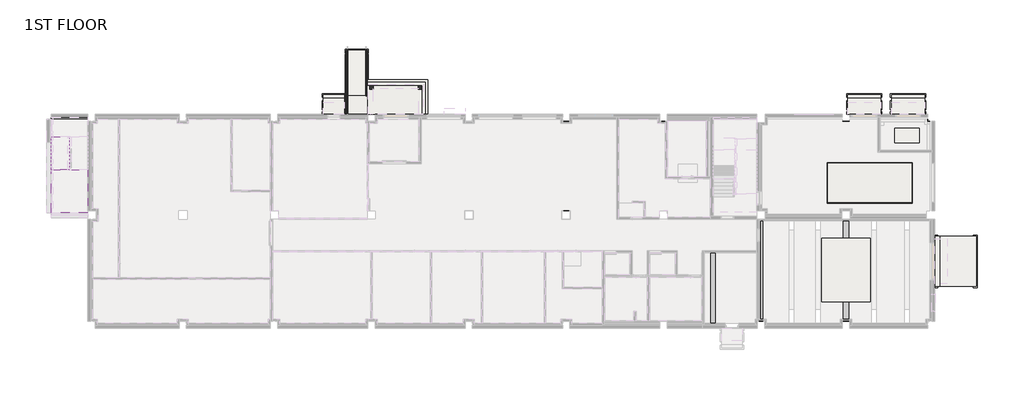
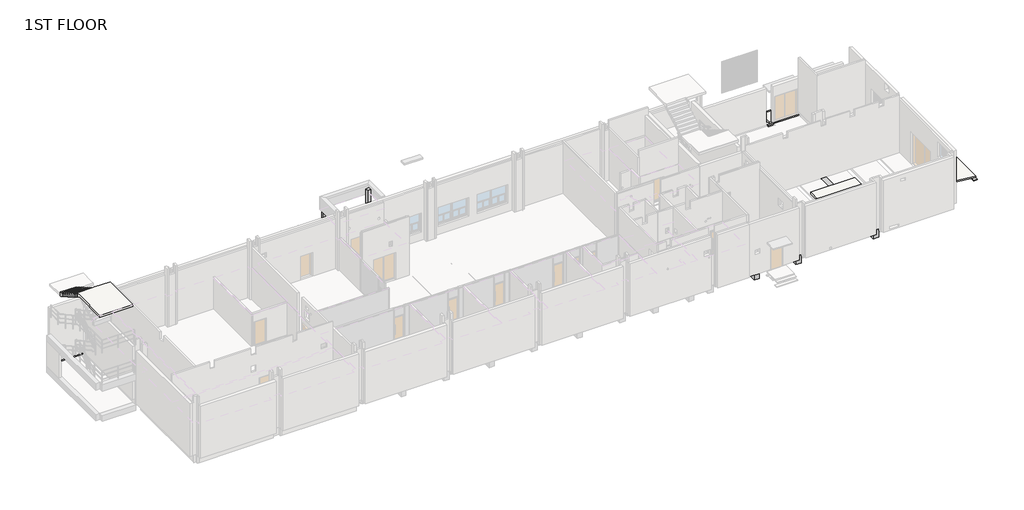
# One storey, part 10 of 15: 37 slabs, 9 beams, 2 columns, 1 stair flight.
"""IFC4 building model written with IfcOpenShell, lengths in millimetres."""

from ifc_helpers import new_model, si_unit, frame, origin, place, context, project, spatial, polyline, outline, extrude, faceted_brep, element, save

model = new_model("IFC4")

# Units and contexts
model_context = context("Model", 3, world=origin())
ifc_project = project(units=[si_unit("LENGTHUNIT", "METRE", prefix="MILLI")], contexts=[model_context])

# Site, building, storey
site = spatial("IfcSite", under=ifc_project)
building = spatial("IfcBuilding", under=site)
storey = spatial("IfcBuildingStorey", under=building, Name="1ST FLOOR", Elevation=4800.0)

# Beams
placement = place(None, origin())
element("IfcBeam", 1, ObjectType="RC Beam_Rectangular : H_SB_AR S16_TG-UG_500x800_1G2A", at=placement, inside=storey, context=model_context, shape_type="Brep", body=[
    faceted_brep([(47350.0, -8350.0, 4800.0), (50825.0, -8350.0, 4800.0), (50825.0, -7850.0, 4800.0), (47350.0, -7850.0, 4800.0), (47350.0, -8350.0, 4650.0), (47350.0, -8350.0, 4000.0), (50825.0, -8350.0, 4000.0), (50825.0, -8350.0, 4650.0), (47350.0, -7850.0, 4000.0), (50825.0, -7850.0, 4000.0), (50825.0, -7850.0, 4650.0), (47350.0, -7850.0, 4650.0)], [[[0, 1, 2, 3]], [[1, 0, 4, 5, 6, 7]], [[6, 5, 8, 9]], [[2, 10, 9, 8, 11, 3]], [[2, 1, 7, 6, 9, 10]], [[8, 5, 4, 0, 3, 11]]]),
])
element("IfcBeam", 2, ObjectType="RC Beam_Rectangular : H_SB_AR S16_TG-UG_500x800_1G1", at=placement, inside=storey, context=model_context, shape_type="Brep", body=[
    faceted_brep([(39250.0, -300.0, 4800.0), (38750.0, -300.0, 4800.0), (38750.0, -7650.0, 4800.0), (39250.0, -7650.0, 4800.0), (39250.0, -7650.0, 4650.0), (39250.0, -7650.0, 4000.0), (39250.0, -300.0, 4000.0), (39250.0, -300.0, 4650.0), (38750.0, -300.0, 4000.0), (38750.0, -7650.0, 4000.0), (38750.0, -300.0, 4650.0), (38750.0, -7650.0, 4650.0)], [[[0, 1, 2, 3]], [[0, 3, 4, 5, 6, 7]], [[8, 6, 5, 9]], [[2, 1, 10, 8, 9, 11]], [[1, 0, 7, 6, 8, 10]], [[3, 2, 11, 9, 5, 4]]]),
])
element("IfcBeam", 3, ObjectType="RC Beam_Rectangular : H_SB_AR S16_TG-UG_500x800_1G1", at=placement, inside=storey, context=model_context, shape_type="Brep", body=[
    faceted_brep([(47300.0, -300.0, 4800.0), (47150.0, -300.0, 4800.0), (46800.0, -300.0, 4800.0), (46800.0, -7650.0, 4800.0), (47300.0, -7650.0, 4800.0), (47300.0, -4975.0, 4800.0), (47300.0, -4825.0, 4800.0), (47300.0, -300.0, 4000.0), (47300.0, -7650.0, 4650.0), (47300.0, -7650.0, 4000.0), (46800.0, -300.0, 4000.0), (46800.0, -7650.0, 4000.0), (46800.0, -300.0, 4650.0), (46800.0, -7650.0, 4650.0)], [[[0, 1, 2, 3, 4, 5, 6]], [[7, 0, 6, 5, 4, 8, 9]], [[10, 7, 9, 11]], [[3, 2, 12, 10, 11, 13]], [[2, 1, 0, 7, 10, 12]], [[4, 3, 13, 11, 9, 8]]]),
])
element("IfcBeam", 4, ObjectType="RC Beam_Rectangular : H_SB_AR S16_TG-UG_450x800_1B1", at=placement, inside=storey, context=model_context, shape_type="Brep", body=[
    faceted_brep([(42125.0, -100.0, 4800.0), (41675.0, -100.0, 4800.0), (41675.0, -7850.0, 4800.0), (42125.0, -7850.0, 4800.0), (42125.0, -7850.0, 4650.0), (42125.0, -7850.0, 4000.0), (42125.0, -100.0, 4000.0), (42125.0, -100.0, 4650.0), (41675.0, -100.0, 4000.0), (41675.0, -7850.0, 4000.0), (41675.0, -100.0, 4650.0), (41675.0, -7850.0, 4650.0)], [[[0, 1, 2, 3]], [[0, 3, 4, 5, 6, 7]], [[8, 6, 5, 9]], [[2, 1, 10, 8, 9, 11]], [[1, 0, 7, 6, 8, 10]], [[3, 2, 11, 9, 5, 4]]]),
])
element("IfcBeam", 5, ObjectType="RC Beam_Rectangular : H_SB_AR S16_TG-UG_450x800_1B1", at=placement, inside=storey, context=model_context, shape_type="Brep", body=[
    faceted_brep([(45325.0, -100.0, 4800.0), (44875.0, -100.0, 4800.0), (44875.0, -7850.0, 4800.0), (45325.0, -7850.0, 4800.0), (45325.0, -7850.0, 4650.0), (45325.0, -7850.0, 4000.0), (45325.0, -100.0, 4000.0), (45325.0, -100.0, 4650.0), (44875.0, -100.0, 4000.0), (44875.0, -7850.0, 4000.0), (44875.0, -100.0, 4650.0), (44875.0, -7850.0, 4650.0)], [[[0, 1, 2, 3]], [[0, 3, 4, 5, 6, 7]], [[8, 6, 5, 9]], [[2, 1, 10, 8, 9, 11]], [[1, 0, 7, 6, 8, 10]], [[3, 2, 11, 9, 5, 4]]]),
])
element("IfcBeam", 6, ObjectType="RC Beam_Rectangular : H_SB_AR S16_TG-UG_450x800_1B1A", at=placement, inside=storey, context=model_context, shape_type="Brep", body=[
    faceted_brep([(50825.0, -8350.0, 4800.0), (51275.0, -8350.0, 4800.0), (51275.0, -8350.0, 4650.0), (51275.0, -8350.0, 4000.0), (50825.0, -8350.0, 4000.0), (50825.0, -8350.0, 4650.0), (50825.0, -16900.0, 4800.0), (51275.0, -16900.0, 4800.0), (51275.0, -16900.0, 4650.0), (51275.0, -16900.0, 4000.0), (50825.0, -16900.0, 4000.0), (50825.0, -15750.0000001, 4000.0), (50825.0, -16900.0, 4650.0)], [[[0, 1, 2, 3, 4, 5]], [[1, 0, 6, 7]], [[1, 7, 8, 9, 3, 2]], [[4, 3, 9, 10, 11]], [[6, 0, 5, 4, 11, 10, 12]], [[7, 6, 12, 10, 9, 8]]]),
])
element("IfcBeam", 7, ObjectType="RC Beam_Rectangular : H_SB_AR S16_TG-UG_500x800_1G1", at=placement, inside=storey, context=model_context, shape_type="Brep", body=[
    faceted_brep([(55200.0, -8350.0, 4800.0), (54700.0, -8350.0, 4800.0), (54700.0, -16700.0, 4800.0), (55200.0, -16700.0, 4800.0), (55200.0, -16700.0, 4650.0), (55200.0, -16700.0, 4000.0), (55200.0, -8350.0, 4000.0), (55200.0, -8350.0, 4650.0), (54700.0, -8350.0, 4000.0), (54700.0, -16700.0, 4000.0), (54700.0, -8350.0, 4650.0), (54700.0, -16700.0, 4650.0)], [[[0, 1, 2, 3]], [[0, 3, 4, 5, 6, 7]], [[8, 6, 5, 9]], [[2, 1, 10, 8, 9, 11]], [[1, 0, 7, 6, 8, 10]], [[3, 2, 11, 9, 5, 4]]]),
])
element("IfcBeam", 8, ObjectType="RC Beam_Rectangular : H_SB_AR S16_TG-UG_500x800_1G1", at=placement, inside=storey, context=model_context, shape_type="Brep", body=[
    faceted_brep([(62250.0, -8350.0, 4800.0), (61750.0, -8350.0, 4800.0), (61750.0, -16700.0, 4800.0), (62250.0, -16700.0, 4800.0), (62250.0, -16700.0, 4650.0), (62250.0, -16700.0, 4000.0), (62250.0, -8350.0, 4000.0), (62250.0, -8350.0, 4650.0), (61750.0, -8350.0, 4000.0), (61750.0, -16700.0, 4000.0), (61750.0, -8350.0, 4650.0), (61750.0, -16700.0, 4650.0)], [[[0, 1, 2, 3]], [[0, 3, 4, 5, 6, 7]], [[8, 6, 5, 9]], [[2, 1, 10, 8, 9, 11]], [[1, 0, 7, 6, 8, 10]], [[3, 2, 11, 9, 5, 4]]]),
])
element("IfcBeam", 9, ObjectType="RC Beam_Rectangular : H_SB_AR S16_RC Beam-AG_400x530_SG1A", at=placement, inside=storey, context=model_context, shape_type="Brep", body=[
    faceted_brep([(-300.0, -100.0, 4630.0), (-300.0, 50.0, 4630.0), (-300.0, 300.0, 4630.0), (-3300.0, 300.0, 4630.0), (-3300.0, 50.0, 4630.0), (-3300.0, -100.0, 4630.0), (-300.0, -100.0, 4100.0), (-300.0, -100.0, 4430.0), (-3300.0, -100.0, 4430.0), (-3300.0, -100.0, 4100.0), (-300.0, 300.0, 4100.0), (-3300.0, 300.0, 4100.0)], [[[0, 1, 2, 3, 4, 5]], [[6, 7, 0, 5, 8, 9]], [[10, 6, 9, 11]], [[2, 10, 11, 3]], [[2, 1, 0, 7, 6, 10]], [[3, 11, 9, 8, 5, 4]]]),
])

# Columns
element("IfcColumn", 10, ObjectType="RC_Column_Rectangular : H_SC_AR S15_RC Col-AG_300x300_C4", at=placement, inside=storey, context=model_context, shape_type="Brep", body=[
    faceted_brep([(23150.0, 2650.0, 4585.0), (23150.0, 2620.0, 4585.0), (23150.0, 2350.0, 4585.0), (22850.0, 2350.0, 4585.0), (22850.0, 2620.0, 4585.0), (22850.0, 2650.0, 4585.0), (23150.0, 2650.0, 9300.0), (23150.0, 2350.0, 9300.0), (23150.0, 2350.0, 4750.0), (22850.0, 2350.0, 9300.0), (22850.0, 2350.0, 4750.0), (22850.0, 2650.0, 9300.0), (23000.0, 2650.0, 9300.0)], [[[0, 1, 2, 3, 4, 5]], [[6, 7, 8, 2, 1, 0]], [[7, 9, 10, 3, 2, 8]], [[9, 11, 5, 4, 3, 10]], [[11, 12, 6, 0, 5]], [[6, 12, 11, 9, 7]]]),
])
element("IfcColumn", 11, ObjectType="RC_Column_Rectangular : H_SC_AR S15_RC Col-AG_300x300_C4", at=placement, inside=storey, context=model_context, shape_type="Brep", body=[
    faceted_brep([(27150.0, 2650.0, 4585.0), (27150.0, 2350.0, 4585.0), (27120.0, 2350.0, 4585.0), (26850.0, 2350.0, 4585.0), (26850.0, 2620.0, 4585.0), (26850.0, 2650.0, 4585.0), (27150.0, 2650.0, 9300.0), (27150.0, 2500.0, 9300.0), (27150.0, 2350.0, 9300.0), (26850.0, 2350.0, 9300.0), (26850.0, 2350.0, 4750.0), (26850.0, 2650.0, 9300.0)], [[[0, 1, 2, 3, 4, 5]], [[6, 7, 8, 1, 0]], [[8, 9, 10, 3, 2, 1]], [[9, 11, 5, 4, 3, 10]], [[11, 6, 0, 5]], [[6, 11, 9, 8, 7]]]),
])

# Slabs
element("IfcSlab", 12, ObjectType="H_SF_AR S18_MAT_T650_MF2", at=placement, inside=storey, context=model_context, shape_type="Brep", body=[
    faceted_brep([(27625.0, 3125.0000075, 4100.0), (27625.0, 300.0, 4100.0), (22650.0, 300.0, 4100.0), (22650.0, 3125.0000075, 4100.0), (22650.0, 300.0, 4750.0), (27120.0, 300.0, 4750.0), (27120.0, 2350.0, 4750.0), (26850.0, 2350.0, 4750.0), (26850.0, 2620.0, 4750.0), (23150.0, 2620.0, 4750.0), (23150.0, 2350.0, 4750.0), (22850.0, 2350.0, 4750.0), (22850.0, 2620.0, 4750.0), (22650.0, 2620.0, 4750.0), (27625.0, 3125.0000075, 4500.0), (27625.0, 300.0, 4500.0), (27420.0, 300.0, 4500.0), (27420.0, 300.0, 4585.0), (27120.0, 300.0, 4585.0), (22650.0, 300.0, 4500.0), (22650.0, 300.0, 4450.0), (22650.0, 300.0, 4400.0), (22650.0, 2620.0, 4585.0), (22650.0, 2920.0, 4585.0), (22650.0, 2920.0, 4500.0), (22650.0, 3125.0000075, 4500.0), (22650.0, 3125.0000075, 4361.6666662), (22650.0, 3125.0000075, 4311.5556782), (27420.0, 2920.0, 4585.0), (22850.0, 2620.0, 4585.0), (22850.0, 2350.0, 4585.0), (23150.0, 2350.0, 4585.0), (23150.0, 2620.0, 4585.0), (26850.0, 2620.0, 4585.0), (26850.0, 2350.0, 4585.0), (27120.0, 2350.0, 4585.0), (27420.0, 2920.0, 4500.0)], [[[0, 1, 2, 3]], [[4, 5, 6, 7, 8, 9, 10, 11, 12, 13]], [[1, 0, 14, 15]], [[2, 1, 15, 16, 17, 18, 5, 4, 19, 20, 21]], [[3, 2, 21, 20, 19, 4, 13, 22, 23, 24, 25, 26, 27]], [[0, 3, 27, 26, 25, 14]], [[17, 28, 23, 22, 29, 30, 31, 32, 33, 34, 35, 18]], [[28, 17, 16, 36]], [[36, 16, 15, 14, 25, 24]], [[5, 18, 35, 6]], [[23, 28, 36, 24]], [[8, 33, 32, 9]], [[22, 13, 12, 29]], [[35, 34, 7, 6]], [[34, 33, 8, 7]], [[32, 31, 10, 9]], [[31, 30, 11, 10]], [[30, 29, 12, 11]]]),
])
element("IfcSlab", 13, ObjectType="H_SF_AR B01_EQ Fdn_T800_EF1", at=placement, inside=storey, context=model_context, shape_type="Brep", body=[
    faceted_brep([(60500.0, -3750.0, 4200.0), (67400.0, -3750.0, 4200.0), (67400.0, -6950.0, 4200.0), (60500.0, -6950.0, 4200.0), (60500.0, -3750.0, 5000.0), (60500.0, -6950.0, 5000.0), (67400.0, -6950.0, 5000.0), (67400.0, -3750.0, 5000.0), (60500.0, -3750.0, 4600.0), (60500.0, -3750.0, 4650.0), (67400.0, -3750.0, 4650.0), (67400.0, -3750.0, 4600.0), (67400.0, -6950.0, 4650.0), (67400.0, -6950.0, 4600.0), (60500.0, -6950.0, 4650.0), (60500.0, -6950.0, 4600.0)], [[[0, 1, 2, 3]], [[4, 5, 6, 7]], [[1, 0, 8, 9, 4, 7, 10, 11]], [[2, 1, 11, 10, 7, 6, 12, 13]], [[3, 2, 13, 12, 6, 5, 14, 15]], [[0, 3, 15, 14, 5, 4, 9, 8]]]),
])
element("IfcSlab", 14, ObjectType="H_SF_AR B01_EQ Fdn_T200_EF2", at=placement, inside=storey, context=model_context, shape_type="SweptSolid", body=[
    extrude(outline(polyline([(64000.0000005, -9900.0), (64000.0000005, -15100.0), (59999.9999995, -15100.0), (59999.9999995, -9900.0), (64000.0000005, -9900.0)])), frame((0.0, 0.0, 4800.0), z_axis=(0.0, 0.0, 1.0), x_axis=(1.0, 0.0, 0.0)), (0.0, 0.0, 1.0), 200.0),
])
element("IfcSlab", 15, ObjectType="H_SF_AR B01_EQ Fdn_T200_EF3", at=placement, inside=storey, context=model_context, shape_type="SweptSolid", body=[
    extrude(outline(polyline([(66000.0, -850.0), (68000.0, -850.0), (68000.0, -2050.0), (66000.0, -2050.0), (66000.0, -850.0)])), frame((0.0, 0.0, 4800.0), z_axis=(0.0, 0.0, 1.0), x_axis=(1.0, 0.0, 0.0)), (0.0, 0.0, 1.0), 200.0),
])
element("IfcSlab", 16, ObjectType="H_FL_AR_S17_RC Slab_T200_SS1", at=placement, inside=storey, context=model_context, shape_type="Brep", body=[
    faceted_brep([(-1850.0, -4250.0, 14050.0), (-3300.0, -4250.0, 14050.0), (-3300.0, -4604.0698283, 14050.0), (-3300.0, -7800.0, 14050.0), (-300.0, -7800.0, 14050.0), (-300.0, -4250.0, 14050.0), (-1750.0, -4250.0, 14050.0), (-1850.0, -4250.0, 13850.0), (-1850.0, -4250.0, 13643.4592668), (-3300.0, -4250.0, 13643.4592668), (-3300.0, -4604.0698283, 13850.0), (-3300.0, -7800.0, 13850.0), (-300.0, -7800.0, 13850.0), (-300.0, -4250.0, 13850.0), (-1750.0, -4250.0, 13850.0), (-1850.0, -4604.0698283, 13850.0)], [[[0, 1, 2, 3, 4, 5, 6]], [[1, 0, 7, 8, 9]], [[1, 9, 10, 11, 3, 2]], [[4, 3, 11, 12]], [[5, 4, 12, 13]], [[0, 6, 14, 7]], [[10, 15, 7, 14, 13, 12, 11]], [[15, 10, 9, 8]], [[7, 15, 8]], [[6, 5, 13, 14]]]),
])
element("IfcSlab", 17, ObjectType="H_SF_AR_B08_Ramp_T150", at=placement, inside=storey, context=model_context, shape_type="SweptSolid", body=[
    extrude(outline(polyline([(69700.0, -9750.0), (69700.0, -13850.0), (69312.0, -13850.0), (69312.0, -9750.0), (69700.0, -9750.0)])), frame((0.0, 0.0, 4650.0), z_axis=(0.0, 0.0, 1.0), x_axis=(1.0, 0.0, 0.0)), (0.0, 0.0, 1.0), 150.0),
])
element("IfcSlab", 18, ObjectType="H_SF_AR_B08_Ramp_T150", at=placement, inside=storey, context=model_context, shape_type="Brep", body=[
    faceted_brep([(72700.0, -9750.0, 4349.2518657), (72700.0, -10050.0, 4349.2518657), (72700.0, -13550.0, 4349.2518657), (72700.0, -13850.0, 4349.2518657), (72256.3868159, -13850.0, 4393.6131841), (72256.3868159, -13550.0, 4393.6131841), (72256.3868159, -10050.0, 4393.6131841), (72256.3868159, -9750.0, 4393.6131841), (69700.0, -10050.0, 4649.2518657), (69700.0, -9750.0, 4649.2518657), (72250.0, -9750.0, 4394.2518657), (72250.0, -10050.0, 4394.2518657), (72250.0, -13550.0, 4394.2518657), (72250.0, -13850.0, 4394.2518657), (69700.0, -13850.0, 4649.2518657), (69700.0, -13550.0, 4649.2518657), (72700.0, -13850.0, 4500.0), (72700.0, -9750.0, 4500.0), (69700.0, -9750.0, 4800.0), (69700.0, -13850.0, 4800.0), (69700.0, -13850.0, 4650.0), (72250.0, -13850.0, 4400.0), (69700.0, -9750.0, 4650.0), (72250.0, -9750.0, 4400.0)], [[[0, 1, 2, 3, 4, 5, 6, 7]], [[8, 9, 10, 11, 12, 13, 14, 15]], [[16, 17, 18, 19]], [[17, 16, 3, 2, 1, 0]], [[16, 19, 20, 14, 13, 21, 4, 3]], [[19, 18, 22, 9, 8, 15, 14, 20]], [[18, 17, 0, 7, 23, 10, 9, 22]], [[21, 23, 7, 6, 5, 4]], [[23, 21, 13, 12, 11, 10]]]),
])
element("IfcSlab", 19, ObjectType="H_SF_AR_S18_Lean_T50", at=placement, inside=storey, context=model_context, shape_type="SweptSolid", body=[
    extrude(outline(polyline([(69550.0, -9650.0), (69550.0, -13950.0), (69300.0, -13950.0), (69300.0, -9650.0), (69550.0, -9650.0)])), frame((0.0, 0.0, 4450.0), z_axis=(0.0, 0.0, 1.0), x_axis=(1.0, 0.0, 0.0)), (0.0, 0.0, 1.0), 50.0),
])
element("IfcSlab", 20, ObjectType="H_SF_AR_S18_Lean_T50", at=placement, inside=storey, context=model_context, shape_type="SweptSolid", body=[
    extrude(outline(polyline([(72450.0, -9650.0), (72800.0, -9650.0), (72800.0, -13950.0), (72450.0, -13950.0), (72450.0, -9650.0)])), frame((0.0, 0.0, 4150.0), z_axis=(0.0, 0.0, 1.0), x_axis=(1.0, 0.0, 0.0)), (0.0, 0.0, 1.0), 50.0),
])
element("IfcSlab", 21, ObjectType="H_SF_AR_S18_Lean_T50", at=placement, inside=storey, context=model_context, shape_type="Brep", body=[
    faceted_brep([(69700.0, -13550.0, 4599.0024876), (69700.0, -10050.0, 4599.0024876), (69717.9210597, -10050.0, 4597.2103816), (72233.6520381, -10050.0, 4345.6372838), (72233.6520381, -13550.0, 4345.6372838), (69717.9210597, -13550.0, 4597.2103816), (69700.0, -10050.0, 4649.2518657), (69700.0, -13550.0, 4649.2518657), (72250.0, -13550.0, 4394.2518657), (72250.0, -10050.0, 4394.2518657), (69700.0, -13550.0, 4600.0), (72229.2893219, -13550.0, 4350.0), (72250.0, -13550.0, 4350.0), (69700.0, -10050.0, 4600.0), (72250.0, -10050.0, 4350.0), (72229.2893219, -10050.0, 4350.0)], [[[0, 1, 2, 3, 4, 5]], [[6, 7, 8, 9]], [[7, 10, 0, 5, 4, 11, 12, 8]], [[1, 0, 10, 7, 6, 13]], [[1, 13, 6, 9, 14, 15, 3, 2]], [[15, 11, 4, 3]], [[11, 15, 14, 12]], [[12, 14, 9, 8]]]),
])
element("IfcSlab", 22, ObjectType="H_SF_AR_B08_Ramp_T150", at=placement, inside=storey, context=model_context, shape_type="Brep", body=[
    faceted_brep([(22638.0, 1800.0, 4600.0), (22638.0, 312.0, 4600.0), (22338.0, 312.0, 4600.0), (21238.0, 312.0, 4600.0), (20938.0, 312.0, 4600.0), (20938.0, 1800.0, 4600.0), (22638.0, 1800.0, 4750.0), (20938.0, 1800.0, 4750.0), (20938.0, 312.0, 4750.0), (22638.0, 312.0, 4750.0)], [[[0, 1, 2, 3, 4, 5]], [[6, 7, 8, 9]], [[1, 0, 6, 9]], [[4, 3, 2, 1, 9, 8]], [[5, 4, 8, 7]], [[0, 5, 7, 6]]]),
])
element("IfcSlab", 23, ObjectType="H_SF_AR_B08_Stoop_T150", at=placement, inside=storey, context=model_context, shape_type="Brep", body=[
    faceted_brep([(68450.0, 1600.0, 4600.0), (68450.0, 1400.0, 4600.0), (68450.0, 662.0000074, 4600.0), (68450.0, 312.0000074, 4600.0), (65750.0, 312.0000074, 4600.0), (65750.0, 662.0000074, 4600.0), (65750.0, 1400.0, 4600.0), (65750.0, 1600.0, 4600.0), (68450.0, 1600.0, 4750.0), (65750.0, 1600.0, 4750.0), (65750.0, 312.0000074, 4750.0), (68450.0, 312.0000074, 4750.0), (68450.0, 1600.0, 4625.0), (65750.0, 1600.0, 4625.0)], [[[0, 1, 2, 3, 4, 5, 6, 7]], [[8, 9, 10, 11]], [[3, 2, 1, 0, 12, 8, 11]], [[4, 3, 11, 10]], [[7, 6, 5, 4, 10, 9, 13]], [[0, 7, 13, 9, 8, 12]]]),
])
element("IfcSlab", 24, ObjectType="H_SF_AR_B08_Stoop_T125", at=placement, inside=storey, context=model_context, shape_type="SweptSolid", body=[
    extrude(outline(polyline([(68450.0, 1900.0), (68450.0, 1600.0), (65750.0, 1600.0), (65750.0, 1900.0), (68450.0, 1900.0)])), frame((0.0, 0.0, 4600.0), z_axis=(0.0, 0.0, 1.0), x_axis=(1.0, 0.0, 0.0)), (0.0, 0.0, 1.0), 25.0),
])
element("IfcSlab", 25, ObjectType="H_SF_AR_S18_Lean_T50", at=placement, inside=storey, context=model_context, shape_type="SweptSolid", body=[
    extrude(outline(polyline([(68550.0, 2000.0), (68550.0, 1700.0), (65650.0, 1700.0), (65650.0, 2000.0), (68550.0, 2000.0)])), frame((0.0, 0.0, 4250.0), z_axis=(0.0, 0.0, 1.0), x_axis=(1.0, 0.0, 0.0)), (0.0, 0.0, 1.0), 50.0),
])
element("IfcSlab", 26, ObjectType="H_SF_AR_S18_Lean_T50", at=placement, inside=storey, context=model_context, shape_type="SweptSolid", body=[
    extrude(outline(polyline([(68550.0, 300.0), (65650.0, 300.0), (65650.0, 512.0000074), (68550.0, 512.0000074), (68550.0, 300.0)])), frame((0.0, 0.0, 4400.0), z_axis=(0.0, 0.0, 1.0), x_axis=(1.0, 0.0, 0.0)), (0.0, 0.0, 1.0), 50.0),
])
element("IfcSlab", 27, ObjectType="H_SF_AR_S18_Lean_T50", at=placement, inside=storey, context=model_context, shape_type="Brep", body=[
    faceted_brep([(68550.0, 1400.0, 4550.0), (68550.0, 1379.2893219, 4550.0), (68550.0, 682.7106855, 4550.0), (68550.0, 662.0000074, 4550.0), (65650.0, 662.0000074, 4550.0), (65650.0, 682.7106855, 4550.0), (65650.0, 1379.2893219, 4550.0), (65650.0, 1400.0, 4550.0), (68550.0, 1400.0, 4600.0), (65650.0, 1400.0, 4600.0), (65650.0, 662.0000074, 4600.0), (68550.0, 662.0000074, 4600.0)], [[[0, 1, 2, 3, 4, 5, 6, 7]], [[8, 9, 10, 11]], [[3, 2, 1, 0, 8, 11]], [[4, 3, 11, 10]], [[7, 6, 5, 4, 10, 9]], [[0, 7, 9, 8]]]),
])
element("IfcSlab", 28, ObjectType="H_SF_AR_B08_Stoop_T150", at=placement, inside=storey, context=model_context, shape_type="Brep", body=[
    faceted_brep([(64850.0, 1600.0, 4600.0), (64850.0, 1400.0, 4600.0), (64850.0, 662.0000074, 4600.0), (64850.0, 312.0000074, 4600.0), (62150.0, 312.0000074, 4600.0), (62150.0, 662.0000074, 4600.0), (62150.0, 1400.0, 4600.0), (62150.0, 1600.0, 4600.0), (64850.0, 1600.0, 4750.0), (62150.0, 1600.0, 4750.0), (62150.0, 312.0000074, 4750.0), (64850.0, 312.0000074, 4750.0), (64850.0, 1600.0, 4625.0), (62150.0, 1600.0, 4625.0)], [[[0, 1, 2, 3, 4, 5, 6, 7]], [[8, 9, 10, 11]], [[3, 2, 1, 0, 12, 8, 11]], [[4, 3, 11, 10]], [[7, 6, 5, 4, 10, 9, 13]], [[0, 7, 13, 9, 8, 12]]]),
])
element("IfcSlab", 29, ObjectType="H_SF_AR_B08_Stoop_T125", at=placement, inside=storey, context=model_context, shape_type="SweptSolid", body=[
    extrude(outline(polyline([(64850.0, 1900.0), (64850.0, 1600.0), (62150.0, 1600.0), (62150.0, 1900.0), (64850.0, 1900.0)])), frame((0.0, 0.0, 4600.0), z_axis=(0.0, 0.0, 1.0), x_axis=(1.0, 0.0, 0.0)), (0.0, 0.0, 1.0), 25.0),
])
element("IfcSlab", 30, ObjectType="H_SF_AR_S18_Lean_T50", at=placement, inside=storey, context=model_context, shape_type="SweptSolid", body=[
    extrude(outline(polyline([(64950.0, 2000.0), (64950.0, 1700.0), (62050.0, 1700.0), (62050.0, 2000.0), (64950.0, 2000.0)])), frame((0.0, 0.0, 4250.0), z_axis=(0.0, 0.0, 1.0), x_axis=(1.0, 0.0, 0.0)), (0.0, 0.0, 1.0), 50.0),
])
element("IfcSlab", 31, ObjectType="H_SF_AR_S18_Lean_T50", at=placement, inside=storey, context=model_context, shape_type="SweptSolid", body=[
    extrude(outline(polyline([(64950.0, 300.0), (62050.0, 300.0), (62050.0, 512.0000074), (64950.0, 512.0000074), (64950.0, 300.0)])), frame((0.0, 0.0, 4400.0), z_axis=(0.0, 0.0, 1.0), x_axis=(1.0, 0.0, 0.0)), (0.0, 0.0, 1.0), 50.0),
])
element("IfcSlab", 32, ObjectType="H_SF_AR_S18_Lean_T50", at=placement, inside=storey, context=model_context, shape_type="Brep", body=[
    faceted_brep([(64950.0, 1400.0, 4550.0), (64950.0, 1379.2893219, 4550.0), (64950.0, 682.7106855, 4550.0), (64950.0, 662.0000074, 4550.0), (62050.0, 662.0000074, 4550.0), (62050.0, 682.7106855, 4550.0), (62050.0, 1379.2893219, 4550.0), (62050.0, 1400.0, 4550.0), (64950.0, 1400.0, 4600.0), (62050.0, 1400.0, 4600.0), (62050.0, 662.0000074, 4600.0), (64950.0, 662.0000074, 4600.0)], [[[0, 1, 2, 3, 4, 5, 6, 7]], [[8, 9, 10, 11]], [[3, 2, 1, 0, 8, 11]], [[4, 3, 11, 10]], [[7, 6, 5, 4, 10, 9]], [[0, 7, 9, 8]]]),
])
element("IfcSlab", 33, ObjectType="H_SF_AR_B08_Stoop_T150", at=placement, inside=storey, context=model_context, shape_type="Brep", body=[
    faceted_brep([(20750.0, 1600.0, 4630.0), (20750.0, 1400.0, 4630.0), (20750.0, 662.0000074, 4630.0), (20750.0, 312.0000074, 4630.0), (19050.0, 312.0000074, 4630.0), (19050.0, 662.0000074, 4630.0), (19050.0, 1400.0, 4630.0), (19050.0, 1600.0, 4630.0), (20750.0, 1600.0, 4780.0), (19050.0, 1600.0, 4780.0), (19050.0, 312.0000074, 4780.0), (20750.0, 312.0000074, 4780.0), (20750.0, 1600.0, 4640.0), (19050.0, 1600.0, 4640.0)], [[[0, 1, 2, 3, 4, 5, 6, 7]], [[8, 9, 10, 11]], [[3, 2, 1, 0, 12, 8, 11]], [[4, 3, 11, 10]], [[7, 6, 5, 4, 10, 9, 13]], [[0, 7, 13, 9, 8, 12]]]),
])
element("IfcSlab", 34, ObjectType="H_SF_AR_B08_Stoop_T125", at=placement, inside=storey, context=model_context, shape_type="Brep", body=[
    faceted_brep([(20750.0, 1900.0, 4515.0), (20750.0, 1600.0, 4515.0), (19050.0, 1600.0, 4515.0), (19050.0, 1900.0, 4515.0), (20750.0, 1900.0, 4640.0), (19050.0, 1900.0, 4640.0), (19050.0, 1600.0, 4640.0), (20750.0, 1600.0, 4640.0), (20750.0, 1600.0, 4630.0), (19050.0, 1600.0, 4630.0)], [[[0, 1, 2, 3]], [[4, 5, 6, 7]], [[1, 0, 4, 7, 8]], [[2, 1, 8, 7, 6, 9]], [[3, 2, 9, 6, 5]], [[0, 3, 5, 4]]]),
])
element("IfcSlab", 35, ObjectType="H_SF_AR_S18_Lean_T50", at=placement, inside=storey, context=model_context, shape_type="SweptSolid", body=[
    extrude(outline(polyline([(20850.0, 2000.0), (20850.0, 1700.0), (18950.0, 1700.0), (18950.0, 2000.0), (20850.0, 2000.0)])), frame((0.0, 0.0, 4280.0), z_axis=(0.0, 0.0, 1.0), x_axis=(1.0, 0.0, 0.0)), (0.0, 0.0, 1.0), 50.0),
])
element("IfcSlab", 36, ObjectType="H_SF_AR_S18_Lean_T50", at=placement, inside=storey, context=model_context, shape_type="Brep", body=[
    faceted_brep([(20850.0, 300.0, 4430.0), (18950.0, 300.0, 4430.0), (18950.0, 512.0000074, 4430.0), (20850.0, 512.0000074, 4430.0), (20850.0, 300.0, 4480.0), (20850.0, 512.0000074, 4480.0), (18950.0, 512.0000074, 4480.0), (18950.0, 300.0, 4480.0), (20850.0, 300.0, 4450.0)], [[[0, 1, 2, 3]], [[4, 5, 6, 7]], [[1, 0, 8, 4, 7]], [[2, 1, 7, 6]], [[3, 2, 6, 5]], [[0, 3, 5, 4, 8]]]),
])
element("IfcSlab", 37, ObjectType="H_SF_AR_S18_Lean_T50", at=placement, inside=storey, context=model_context, shape_type="Brep", body=[
    faceted_brep([(20850.0, 1400.0, 4580.0), (20850.0, 1379.2893219, 4580.0), (20850.0, 682.7106855, 4580.0), (20850.0, 662.0000074, 4580.0), (18950.0, 662.0000074, 4580.0), (18950.0, 682.7106855, 4580.0), (18950.0, 1379.2893219, 4580.0), (18950.0, 1400.0, 4580.0), (20850.0, 1400.0, 4630.0), (18950.0, 1400.0, 4630.0), (18950.0, 662.0000074, 4630.0), (20850.0, 662.0000074, 4630.0)], [[[0, 1, 2, 3, 4, 5, 6, 7]], [[8, 9, 10, 11]], [[3, 2, 1, 0, 8, 11]], [[4, 3, 11, 10]], [[7, 6, 5, 4, 10, 9]], [[0, 7, 9, 8]]]),
])
element("IfcSlab", 38, ObjectType="H_SF_AR_B08_Ramp_T150", at=placement, inside=storey, context=model_context, shape_type="Brep", body=[
    faceted_brep([(22638.0, 5550.0, 4349.6670362), (22638.0, 5100.0, 4379.6670362), (22638.0, 1800.0, 4599.6670362), (22338.0, 1800.0, 4599.6670362), (21238.0, 1800.0, 4599.6670362), (20938.0, 1800.0, 4599.6670362), (20938.0, 5100.0, 4379.6670362), (20938.0, 5550.0, 4349.6670362), (22638.0, 5550.0, 4500.0), (20938.0, 5550.0, 4500.0), (20938.0, 1800.0, 4750.0), (22638.0, 1800.0, 4750.0), (22638.0, 1800.0, 4600.0), (20938.0, 1800.0, 4600.0)], [[[0, 1, 2, 3, 4, 5, 6, 7]], [[8, 9, 10, 11]], [[2, 1, 0, 8, 11, 12]], [[5, 4, 3, 2, 12, 11, 10, 13]], [[7, 6, 5, 13, 10, 9]], [[0, 7, 9, 8]]]),
])
element("IfcSlab", 39, ObjectType="H_SF_AR_S18_Lean_T50", at=placement, inside=storey, context=model_context, shape_type="SweptSolid", body=[
    extrude(outline(polyline([(22488.0, 300.0), (21088.0, 300.0), (21088.0, 550.0), (22488.0, 550.0), (22488.0, 300.0)])), frame((0.0, 0.0, 4400.0), z_axis=(0.0, 0.0, 1.0), x_axis=(1.0, 0.0, 0.0)), (0.0, 0.0, 1.0), 50.0),
])
element("IfcSlab", 40, ObjectType="H_SF_AR_S18_Lean_T50", at=placement, inside=storey, context=model_context, shape_type="SweptSolid", body=[
    extrude(outline(polyline([(22738.0, 5650.0), (22738.0, 5300.0), (20838.0, 5300.0), (20838.0, 5650.0), (22738.0, 5650.0)])), frame((0.0, 0.0, 4129.6670362), z_axis=(0.0, 0.0, 1.0), x_axis=(1.0, 0.0, 0.0)), (0.0, 0.0, 1.0), 50.0),
])
element("IfcSlab", 41, ObjectType="H_SF_AR_S18_Lean_T50", at=placement, inside=storey, context=model_context, shape_type="Brep", body=[
    faceted_brep([(22338.0, 1800.0, 4550.0), (22338.0, 700.0, 4550.0), (21238.0, 700.0, 4550.0), (21238.0, 1800.0, 4550.0), (22338.0, 1800.0, 4600.0), (21238.0, 1800.0, 4600.0), (21238.0, 700.0, 4600.0), (22338.0, 700.0, 4600.0), (22338.0, 1800.0, 4599.6670362), (21238.0, 1800.0, 4599.6670362)], [[[0, 1, 2, 3]], [[4, 5, 6, 7]], [[1, 0, 8, 4, 7]], [[2, 1, 7, 6]], [[3, 2, 6, 5, 9]], [[0, 3, 9, 5, 4, 8]]]),
])
element("IfcSlab", 42, ObjectType="H_SF_AR_S18_Lean_T50", at=placement, inside=storey, context=model_context, shape_type="Brep", body=[
    faceted_brep([(20850.0, 1800.0, 4400.0), (21088.0, 1800.0, 4400.0), (21088.0, 550.0, 4400.0), (21088.0, 300.0, 4400.0), (20850.0, 300.0, 4400.0), (21088.0, 1800.0, 4450.0), (20850.0, 1800.0, 4450.0), (20850.0, 300.0, 4450.0), (21088.0, 300.0, 4450.0), (21088.0, 550.0, 4450.0), (20850.0, 300.0, 4430.0)], [[[0, 1, 2, 3, 4]], [[5, 6, 7, 8, 9]], [[1, 0, 6, 5]], [[1, 5, 9, 8, 3, 2]], [[4, 3, 8, 7, 10]], [[0, 4, 10, 7, 6]]]),
    faceted_brep([(22650.0, 1800.0, 4400.0), (22650.0, 300.0, 4400.0), (22488.0, 300.0, 4400.0), (22488.0, 550.0, 4400.0), (22488.0, 1800.0, 4400.0), (22650.0, 300.0, 4450.0), (22650.0, 1800.0, 4450.0), (22488.0, 1800.0, 4450.0), (22488.0, 550.0, 4450.0), (22488.0, 300.0, 4450.0)], [[[0, 1, 2, 3, 4]], [[5, 6, 7, 8, 9]], [[1, 0, 6, 5]], [[2, 1, 5, 9]], [[2, 9, 8, 7, 4, 3]], [[0, 4, 7, 6]]]),
])
element("IfcSlab", 43, ObjectType="H_SF_AR_S18_Lean_T50", at=placement, inside=storey, context=model_context, shape_type="Brep", body=[
    faceted_brep([(22738.0, 5238.2864422, 4170.6699159), (22738.0, 3125.0000075, 4311.5556782), (22650.0, 3125.0000075, 4311.5556782), (22650.0, 1800.0, 4399.8890121), (22488.0, 1800.0, 4399.8890121), (22488.0, 5238.2864422, 4170.6699159), (22488.0, 1800.0, 4450.0), (22650.0, 1800.0, 4450.0), (22650.0, 3125.0000075, 4361.6666662), (22738.0, 3125.0000075, 4361.6666662), (22738.0, 5184.596098, 4224.3602601), (22638.0, 5184.596098, 4224.3602601), (22488.0, 5184.596098, 4224.3602601)], [[[0, 1, 2, 3, 4, 5]], [[6, 7, 8, 9, 10, 11, 12]], [[1, 0, 10, 9]], [[4, 3, 7, 6]], [[5, 4, 6, 12]], [[0, 5, 12, 11, 10]], [[2, 1, 9, 8]], [[3, 2, 8, 7]]]),
    faceted_brep([(21088.0, 1800.0, 4399.8890121), (20850.0, 1800.0, 4399.8890121), (20850.0, 5238.2864422, 4170.6699159), (21088.0, 5238.2864422, 4170.6699159), (20850.0, 1800.0, 4450.0), (21088.0, 1800.0, 4450.0), (21088.0, 5184.596098, 4224.3602601), (20938.0, 5184.596098, 4224.3602601), (20850.0, 5184.596098, 4224.3602601)], [[[0, 1, 2, 3]], [[4, 5, 6, 7, 8]], [[1, 0, 5, 4]], [[2, 1, 4, 8]], [[0, 3, 6, 5]], [[3, 2, 8, 7, 6]]]),
])
element("IfcSlab", 44, ObjectType="H_SF_AR_S18_Lean_T50", at=placement, inside=storey, context=model_context, shape_type="Brep", body=[
    faceted_brep([(65557.0, -1062.0, 4600.0), (65557.0, -100.0, 4600.0), (65577.7106781, -100.0, 4600.0), (68700.0, -100.0, 4600.0), (68700.0, -300.0, 4600.0), (68900.0, -300.0, 4600.0), (68900.0, -2372.2893219, 4600.0), (68900.0, -2393.0, 4600.0), (65057.0, -2393.0, 4600.0), (65057.0, -1082.7106781, 4600.0), (65057.0, -1062.0, 4600.0), (65077.7106781, -1062.0, 4600.0), (65057.0, -1062.0, 4650.0), (65057.0, -2393.0, 4650.0), (68900.0, -2393.0, 4650.0), (68900.0, -300.0, 4650.0), (68700.0, -300.0, 4650.0), (68700.0, -100.0, 4650.0), (65557.0, -100.0, 4650.0), (65557.0, -1062.0, 4650.0)], [[[0, 1, 2, 3, 4, 5, 6, 7, 8, 9, 10, 11]], [[12, 13, 14, 15, 16, 17, 18, 19]], [[13, 12, 10, 9, 8]], [[12, 19, 0, 11, 10]], [[1, 0, 19, 18]], [[18, 17, 3, 2, 1]], [[4, 3, 17, 16]], [[5, 4, 16, 15]], [[15, 14, 7, 6, 5]], [[8, 7, 14, 13]]]),
])
element("IfcSlab", 45, ObjectType="H_SF_AR_S18_Lean_T50", at=placement, inside=storey, context=model_context, shape_type="Brep", body=[
    faceted_brep([(64357.0, -3093.0, 4600.0), (68900.0, -3093.0, 4600.0), (68900.0, -3113.7106781, 4600.0), (68900.0, -7650.0, 4600.0), (68600.0, -7650.0, 4600.0), (68600.0, -7950.0, 4600.0), (62350.0, -7950.0, 4600.0), (62350.0, -7650.0, 4600.0), (61650.0, -7650.0, 4600.0), (61650.0, -7950.0, 4600.0), (55350.0, -7950.0, 4600.0), (55350.0, -7650.0, 4600.0), (55050.0, -7650.0, 4600.0), (55050.0, -400.0, 4600.0), (55350.0, -400.0, 4600.0), (55350.0, -100.0, 4600.0), (61700.0, -100.0, 4600.0), (61700.0, -300.0, 4600.0), (62300.0, -300.0, 4600.0), (62300.0, -100.0, 4600.0), (64357.0, -100.0, 4600.0), (64357.0, -912.0, 4600.0), (64357.0, -1062.0, 4600.0), (64357.0, -1082.7106781, 4600.0), (67400.0, -3750.0, 4600.0), (60500.0, -3750.0, 4600.0), (60500.0, -6950.0, 4600.0), (67400.0, -6950.0, 4600.0), (68900.0, -3093.0, 4650.0), (64357.0, -3093.0, 4650.0), (64357.0, -912.0, 4650.0), (64357.0, -100.0, 4650.0), (62300.0, -100.0, 4650.0), (62300.0, -300.0, 4650.0), (61700.0, -300.0, 4650.0), (61700.0, -100.0, 4650.0), (55350.0, -100.0, 4650.0), (55350.0, -400.0, 4650.0), (55050.0, -400.0, 4650.0), (55050.0, -7650.0, 4650.0), (55350.0, -7650.0, 4650.0), (55350.0, -7950.0, 4650.0), (61650.0, -7950.0, 4650.0), (61650.0, -7650.0, 4650.0), (62350.0, -7650.0, 4650.0), (62350.0, -7950.0, 4650.0), (68600.0, -7950.0, 4650.0), (68600.0, -7650.0, 4650.0), (68900.0, -7650.0, 4650.0), (60500.0, -3750.0, 4650.0), (67400.0, -3750.0, 4650.0), (67400.0, -6950.0, 4650.0), (60500.0, -6950.0, 4650.0)], [[[0, 1, 2, 3, 4, 5, 6, 7, 8, 9, 10, 11, 12, 13, 14, 15, 16, 17, 18, 19, 20, 21, 22, 23], [24, 25, 26, 27]], [[28, 29, 30, 31, 32, 33, 34, 35, 36, 37, 38, 39, 40, 41, 42, 43, 44, 45, 46, 47, 48], [49, 50, 51, 52]], [[1, 0, 29, 28]], [[28, 48, 3, 2, 1]], [[4, 3, 48, 47]], [[5, 4, 47, 46]], [[6, 5, 46, 45]], [[7, 6, 45, 44]], [[8, 7, 44, 43]], [[9, 8, 43, 42]], [[10, 9, 42, 41]], [[11, 10, 41, 40]], [[12, 11, 40, 39]], [[13, 12, 39, 38]], [[14, 13, 38, 37]], [[15, 14, 37, 36]], [[16, 15, 36, 35]], [[17, 16, 35, 34]], [[18, 17, 34, 33]], [[19, 18, 33, 32]], [[20, 19, 32, 31]], [[20, 31, 30, 29, 0, 23, 22, 21]], [[25, 24, 50, 49]], [[26, 25, 49, 52]], [[27, 26, 52, 51]], [[24, 27, 51, 50]]]),
])
element("IfcSlab", 46, ObjectType="H_SF_AR_S18_Lean_T50", at=placement, inside=storey, context=model_context, shape_type="SweptSolid", body=[
    extrude(outline(polyline([(65257.0, -762.0), (64657.0, -762.0), (64657.0, -100.0), (65257.0, -100.0), (65257.0, -762.0)])), frame((0.0, 0.0, 4300.0), z_axis=(0.0, 0.0, 1.0), x_axis=(1.0, 0.0, 0.0)), (0.0, 0.0, 1.0), 50.0),
])
element("IfcSlab", 47, ObjectType="H_SF_AR_S18_Lean_T50", at=placement, inside=storey, context=model_context, shape_type="Brep", body=[
    faceted_brep([(64907.0, -2543.0, 4450.0), (68900.0, -2543.0, 4450.0), (68900.0, -2943.0, 4450.0), (64507.0, -2943.0, 4450.0), (64507.0, -932.7106781, 4450.0), (64907.0, -932.7106781, 4450.0), (68900.0, -2543.0, 4500.0), (64907.0, -2543.0, 4500.0), (64907.0, -982.7106781, 4500.0), (64507.0, -982.7106781, 4500.0), (64507.0, -2943.0, 4500.0), (68900.0, -2943.0, 4500.0)], [[[0, 1, 2, 3, 4, 5]], [[6, 7, 8, 9, 10, 11]], [[7, 0, 5, 8]], [[1, 0, 7, 6]], [[2, 1, 6, 11]], [[3, 2, 11, 10]], [[3, 10, 9, 4]], [[5, 4, 9, 8]]]),
])
element("IfcSlab", 48, ObjectType="H_SF_AR_S18_Lean_T50", at=placement, inside=storey, context=model_context, shape_type="SweptSolid", body=[
    extrude(outline(polyline([(67500.0, -3650.0), (67500.0, -7050.0), (60400.0, -7050.0), (60400.0, -3650.0), (67500.0, -3650.0)])), frame((0.0, 0.0, 4150.0), z_axis=(0.0, 0.0, 1.0), x_axis=(1.0, 0.0, 0.0)), (0.0, 0.0, 1.0), 50.0),
])

# Stair flight
element("IfcStairFlight", 49, ObjectType="Concrete", at=placement, inside=storey, context=model_context, shape_type="Brep", body=[
    faceted_brep([(-1850.0, -1550.0, 12475.0), (-3300.0, -1550.0, 12475.0), (-3300.0, -1604.0698283, 12475.0), (-3300.0, -1850.0, 12475.0), (-1850.0, -1850.0, 12475.0), (-1850.0, -1604.0698283, 12475.0), (-1850.0, -1850.0, 12243.4592668), (-1850.0, -1604.0698283, 12100.0), (-1850.0, -1550.0, 12100.0), (-3300.0, -1550.0, 12100.0), (-3300.0, -1604.0698283, 12100.0), (-3300.0, -1850.0, 12243.4592668), (-1850.0, -2150.0, 12418.4592668), (-1850.0, -2450.0, 12593.4592668), (-1850.0, -2750.0, 12768.4592668), (-1850.0, -3050.0, 12943.4592668), (-1850.0, -3350.0, 13118.4592668), (-1850.0, -3650.0, 13293.4592668), (-1850.0, -3950.0, 13468.4592668), (-1850.0, -4250.0, 13643.4592668), (-3300.0, -4250.0, 13643.4592668), (-3300.0, -3950.0, 13468.4592668), (-3300.0, -3650.0, 13293.4592668), (-3300.0, -3350.0, 13118.4592668), (-3300.0, -3050.0, 12943.4592668), (-3300.0, -2750.0, 12768.4592668), (-3300.0, -2450.0, 12593.4592668), (-3300.0, -2150.0, 12418.4592668), (-1850.0, -2150.0, 12650.0), (-1850.0, -1850.0, 12650.0), (-3300.0, -1850.0, 12650.0), (-3300.0, -2150.0, 12650.0), (-1850.0, -2450.0, 12825.0), (-1850.0, -2150.0, 12825.0), (-3300.0, -2150.0, 12825.0), (-3300.0, -2450.0, 12825.0), (-1850.0, -2750.0, 13000.0), (-1850.0, -2450.0, 13000.0), (-3300.0, -2450.0, 13000.0), (-3300.0, -2750.0, 13000.0), (-1850.0, -3050.0, 13175.0), (-1850.0, -2750.0, 13175.0), (-3300.0, -2750.0, 13175.0), (-3300.0, -3050.0, 13175.0), (-1850.0, -3350.0, 13350.0), (-1850.0, -3050.0, 13350.0), (-3300.0, -3050.0, 13350.0), (-3300.0, -3350.0, 13350.0), (-1850.0, -3650.0, 13525.0), (-1850.0, -3350.0, 13525.0), (-3300.0, -3350.0, 13525.0), (-3300.0, -3650.0, 13525.0), (-1850.0, -3950.0, 13700.0), (-1850.0, -3650.0, 13700.0), (-3300.0, -3650.0, 13700.0), (-3300.0, -3950.0, 13700.0), (-1850.0, -4250.0, 13875.0), (-1850.0, -3950.0, 13875.0), (-3300.0, -3950.0, 13875.0), (-3300.0, -4250.0, 13875.0), (-1850.0, -4250.0, 13850.0)], [[[0, 1, 2, 3, 4, 5]], [[4, 6, 7, 8, 0, 5]], [[1, 0, 8, 9]], [[1, 9, 10, 11, 3, 2]], [[10, 7, 6, 12, 13, 14, 15, 16, 17, 18, 19, 20, 21, 22, 23, 24, 25, 26, 27, 11]], [[7, 10, 9, 8]], [[28, 29, 30, 31]], [[29, 28, 12, 6, 4]], [[30, 29, 4, 3]], [[31, 30, 3, 11, 27]], [[32, 33, 34, 35]], [[33, 32, 13, 12, 28]], [[34, 33, 28, 31]], [[35, 34, 31, 27, 26]], [[36, 37, 38, 39]], [[37, 36, 14, 13, 32]], [[38, 37, 32, 35]], [[39, 38, 35, 26, 25]], [[40, 41, 42, 43]], [[41, 40, 15, 14, 36]], [[42, 41, 36, 39]], [[43, 42, 39, 25, 24]], [[44, 45, 46, 47]], [[45, 44, 16, 15, 40]], [[46, 45, 40, 43]], [[47, 46, 43, 24, 23]], [[48, 49, 50, 51]], [[49, 48, 17, 16, 44]], [[50, 49, 44, 47]], [[51, 50, 47, 23, 22]], [[52, 53, 54, 55]], [[53, 52, 18, 17, 48]], [[54, 53, 48, 51]], [[55, 54, 51, 22, 21]], [[56, 57, 58, 59]], [[57, 56, 60, 19, 18, 52]], [[58, 57, 52, 55]], [[59, 58, 55, 21, 20]], [[56, 59, 20, 19, 60]]]),
])

save(model, "model.ifc")

# Revit data of these elements
# Type "RC Beam_Rectangular : H_SB_AR S16_TG-UG_500x800_1G2A"
#   Type Comments = "CV-UG"
#   중앙부 하부근 = ""
#   중앙부 상부근 = ""
#   중앙부 보조근 = ""
#   중앙부 늑근 = ""
#   외단부 하부근 = ""
#   외단부 상부근 = ""
#   외단부 보조근 = ""
#   외단부 늑근 = ""
#   부호 = "TG3"
#   내단부 하부근 = ""
#   내단부 상부근 = ""
#   내단부 보조근 = ""
#   내단부 늑근 = ""
#   ALL 하부근 = "3-D20"
#   ALL 상부근 = "3-D20"
#   ALL 보조근 = ""
#   ALL 늑근 = "2-D10 @120"
#   H_Rebar Ratio = 0.14
#   Width = 500 mm
#   Height = 800 mm
#   Length [instance default] = 1524 mm
#   b = 500 mm
#   h = 800 mm
#   hec_material3 [instance default] = none
#   hec_material2 [instance default] = none
#   hec_material1 [instance default] = none
#   Structural Material [instance default] = none
#   Assembly Code = ""
# Type "RC Beam_Rectangular : H_SB_AR S16_TG-UG_500x800_1G1"
#   Type Comments = "CV-UG"
#   중앙부 하부근 = ""
#   중앙부 상부근 = ""
#   중앙부 보조근 = ""
#   중앙부 늑근 = ""
#   외단부 하부근 = ""
#   외단부 상부근 = ""
#   외단부 보조근 = ""
#   외단부 늑근 = ""
#   부호 = "TG3"
#   내단부 하부근 = ""
#   내단부 상부근 = ""
#   내단부 보조근 = ""
#   내단부 늑근 = ""
#   ALL 하부근 = "3-D20"
#   ALL 상부근 = "3-D20"
#   ALL 보조근 = ""
#   ALL 늑근 = "2-D10 @120"
#   H_Rebar Ratio = 0.14
#   Width = 500 mm
#   Height = 800 mm
#   Length [instance default] = 1524 mm
#   b = 500 mm
#   h = 800 mm
#   hec_material3 [instance default] = none
#   hec_material2 [instance default] = none
#   hec_material1 [instance default] = none
#   Structural Material [instance default] = none
#   Assembly Code = ""
# Type "RC Beam_Rectangular : H_SB_AR S16_TG-UG_450x800_1B1"
#   Type Comments = "CV-UG"
#   중앙부 하부근 = ""
#   중앙부 상부근 = ""
#   중앙부 보조근 = ""
#   중앙부 늑근 = ""
#   외단부 하부근 = ""
#   외단부 상부근 = ""
#   외단부 보조근 = ""
#   외단부 늑근 = ""
#   부호 = "TG3"
#   내단부 하부근 = ""
#   내단부 상부근 = ""
#   내단부 보조근 = ""
#   내단부 늑근 = ""
#   ALL 하부근 = "3-D20"
#   ALL 상부근 = "3-D20"
#   ALL 보조근 = ""
#   ALL 늑근 = "2-D10 @120"
#   H_Rebar Ratio = 0.14
#   Width = 450 mm
#   Height = 800 mm
#   Length [instance default] = 1524 mm
#   b = 450 mm
#   h = 800 mm
#   hec_material3 [instance default] = none
#   hec_material2 [instance default] = none
#   hec_material1 [instance default] = none
#   Structural Material [instance default] = none
#   Assembly Code = ""
# Type "RC Beam_Rectangular : H_SB_AR S16_TG-UG_450x800_1B1A"
#   Type Comments = "CV-UG"
#   중앙부 하부근 = ""
#   중앙부 상부근 = ""
#   중앙부 보조근 = ""
#   중앙부 늑근 = ""
#   외단부 하부근 = ""
#   외단부 상부근 = ""
#   외단부 보조근 = ""
#   외단부 늑근 = ""
#   부호 = "TG3"
#   내단부 하부근 = ""
#   내단부 상부근 = ""
#   내단부 보조근 = ""
#   내단부 늑근 = ""
#   ALL 하부근 = "3-D20"
#   ALL 상부근 = "3-D20"
#   ALL 보조근 = ""
#   ALL 늑근 = "2-D10 @120"
#   H_Rebar Ratio = 0.14
#   Width = 450 mm
#   Height = 800 mm
#   Length [instance default] = 1524 mm
#   b = 450 mm
#   h = 800 mm
#   hec_material3 [instance default] = none
#   hec_material2 [instance default] = none
#   hec_material1 [instance default] = none
#   Structural Material [instance default] = none
#   Assembly Code = ""
# Type "RC Beam_Rectangular : H_SB_AR S16_RC Beam-AG_400x530_SG1A"
#   Type Comments = "CV-AG"
#   중앙부 하부근 = ""
#   중앙부 상부근 = ""
#   중앙부 보조근 = ""
#   중앙부 늑근 = ""
#   외단부 하부근 = ""
#   외단부 상부근 = ""
#   외단부 보조근 = ""
#   외단부 늑근 = ""
#   부호 = "TG3"
#   내단부 하부근 = ""
#   내단부 상부근 = ""
#   내단부 보조근 = ""
#   내단부 늑근 = ""
#   ALL 하부근 = "3-D20"
#   ALL 상부근 = "3-D20"
#   ALL 보조근 = ""
#   ALL 늑근 = "2-D10 @120"
#   H_Rebar Ratio = 0.14
#   Width = 400 mm
#   Height = 530 mm
#   Length [instance default] = 1524 mm
#   b = 400 mm
#   h = 530 mm
#   hec_material3 [instance default] = none
#   hec_material2 [instance default] = none
#   hec_material1 [instance default] = none
#   Structural Material [instance default] = none
#   Assembly Code = ""
# Type "RC_Column_Rectangular : H_SC_AR S15_RC Col-AG_300x300_C4"
#   Type Comments = "CV-AG"
#   H_Rebar Ratio = 0.3
#   Width = 300 mm
#   Depth = 300 mm
#   hec_material3 [instance default] = none
#   hec_material2 [instance default] = none
#   hec_material1 [instance default] = none
#   Structural Material [instance default] = none
#   Description = (empty or 0)
# Type "H_SF_AR S18_MAT_T650_MF2"
#   Type Comments = "CV-AG"
#   H_Rebar Ratio = 0.12
#   Layers, outside or top first: 650 mm "Concrete_f'c=28MPa(Cylender)" (function 1)
# Type "H_SF_AR B01_EQ Fdn_T800_EF1"
#   Type Comments = "CV-AG"
#   H_Rebar Ratio = 0.12
#   Layers, outside or top first: 800 mm "Concrete_f'c=28MPa(Cylender)" (function 1)
# Type "H_SF_AR B01_EQ Fdn_T200_EF2"
#   Type Comments = "CV-AG"
#   H_Rebar Ratio = 0.12
#   Layers, outside or top first: 200 mm "Concrete_f'c=28MPa(Cylender)" (function 1)
# Type "H_SF_AR B01_EQ Fdn_T200_EF3"
#   Type Comments = "CV-AG"
#   H_Rebar Ratio = 0.12
#   Layers, outside or top first: 200 mm "Concrete_f'c=28MPa(Cylender)" (function 1)
# Type "H_FL_AR_S17_RC Slab_T200_SS1"
#   Type Comments = "CV-AG"
#   H_Rebar Ratio = 0.1
# Type "H_SF_AR_B08_Ramp_T150"
#   Type Comments = "CV-AG"
#   H_Q'ty Cal Type Tag = "SF-Q2"
#   H_WM Code_1 = "A04AS173-00001 |  | M2 | Finishing Work | Exterior/Interior Finish Work | Steel Trowel Finish |  |  |  |  | A04AS173-00001 Finishing Work Exterior/Interior Finish Work Steel Trowel Finish         |"
#   H_WM Code_2 = "A03AD032-00022 |  | M3 | Concrete Work | Substructure Work | Structural Concrete | Cement Type-1 | 25MPa ≤ F'c (Cylinder Strength) < 30MPa |  |  |  |  | A03AD032-00022 Concrete Work Substructure Work Structural Concrete  Cement Type-1 25MPa ≤ F'c (Cylinder Strength) < 30MPa      |  F'c (Cylinder Strength) = 24MPa"
#   H_WM Code_3 = "A03AD037-00002 |  | TON | Concrete Work | Substructure Work | Rebar Work | Deformed Bar (Non-Coat.) | 400MPa<Fy≤470MPa |  |  |  |  | A03AD037-00002 Concrete Work Substructure Work Rebar Work Deformed Bar (Non-Coat.)  400MPa<Fy≤470MPa      | ASTM A615 GRADE 60 (Fy=420MPa)"
#   H_WM Code_4 = "A03AD035-00001 |  | M2 | Concrete Work | Substructure Work | Form Work (3 times in use) | Flat Form | Dressed Lumber, Plywood or Steel Form(Wood Planks are not Allowed) incl. Chamfer |  |  |  | A03AD035-00001 Concrete Work Substructure Work Form Work (3 times in use) Flat Form     Dressed Lumber, Plywood or Steel Form(Wood Planks are not Allowed) incl. Chamfer   |"
#   H_WM Code_5 = "A01ZZ001-00012 |  | M3 | Earth Work | - | Excavation | Soil, Mech. |  | Manual Excavation Above GWL |  |  |  | A01ZZ001-00012 Earth Work - Excavation Soil, Mech.      Manual Excavation Above GWL  | Above GWL"
#   H_WM Code_6 = "A01ZZ001-00013 |  | M3 | Earth Work | - | Excavation | Soil, Mech. |  | Manual Excavation Below GWL |  |  |  | A01ZZ001-00013 Earth Work - Excavation Soil, Mech.      Manual Excavation Below GWL  | Below GWL"
#   H_WM Code_7 = "A01ZZ003-00001 |  | M3 | Earth Work | - | Backfill | Re-use, Soil |  |  |  | Compaction=(  )% |  | A01ZZ003-00001 Earth Work - Backfill Re-use, Soil        | Compaction=( 95 )%"
#   H_WM Code_8 = "A01ZZ004-00001 |  | M3 | Earth Work | - | Disposal | Soil |  |  |  | Disposal Distance=Appx. (  )km from Site |  | A01ZZ004-00001 Earth Work - Disposal Soil        | Disposal Distance=Appx. (20 )km from Site"
#   H_WM Code_9 = "A03AH056-00001 |  | M2 | Concrete Work | Concrete Protective Coating (U/G) | Bitumen/Bituminous/Asphalt Coating |  |  | A03AH056-00001 Concrete Work Concrete Protective Coating (U/G) Bitumen/Bituminous/Asphalt Coating         | *기초바닥 Protection 은 Lean에 적용"
#   H_WM Code_10 = "A03AD034-00013 |  | M3 | Concrete Work | Substructure Work | Lean Concrete (including Form work) | Cement Type-1 | 10MPa ≤ F'c (Cylinder Strength) < 15MPa |  |  | A03AD034-00013 Concrete Work Substructure Work Lean Concrete (including Form work)  Cement Type-1 10MPa ≤ F'c (Cylinder Strength) < 15MPa      | Disposal Distance=Appx. (20 )km from Site"
#   H_Rebar Ratio = 0.1
#   Layers, outside or top first: 150 mm "Concrete_f'c=28MPa(Cylender)" (function 1)
# Type "H_SF_AR_S18_Lean_T50"
#   Type Comments = "Lean"
#   Layers, outside or top first: 50 mm "Concrete_f'c=14MPa(Cylender)" (function 1)
# Type "H_SF_AR_B08_Stoop_T150"
#   Type Comments = "CV-AG"
#   H_Rebar Ratio = 0.1
#   Layers, outside or top first: 150 mm "Concrete_f'c=28MPa(Cylender)" (function 1)
# Type "H_SF_AR_B08_Stoop_T125"
#   Type Comments = "CV-AG"
#   H_Rebar Ratio = 0.1
#   Layers, outside or top first: 125 mm "Concrete_f'c=28MPa(Cylender)" (function 1)
# Type "Concrete"
#   Type Comments = "CV-AG"
#   H_Rebar Ratio = 0.1
# Element 1 (IfcBeam, "RC Beam_Rectangular : H_SB_AR S16_TG-UG_500x800_1G2A")
#   Comments = ""
#   hec_material3 = none
#   hec_material2 = none
#   hec_material1 = none
#   Structural Material = Concrete_f'c=28MPa(Cylender)
#   Phase Created = New Construction
#   Materials on its faces: "Concrete_f'c=28MPa(Cylender)"
# Elements 2, 3, 7, 8 (IfcBeam, "RC Beam_Rectangular : H_SB_AR S16_TG-UG_500x800_1G1")
#   Comments = ""
#   hec_material3 = none
#   hec_material2 = none
#   hec_material1 = none
#   Structural Material = Concrete_f'c=28MPa(Cylender)
#   Phase Created = New Construction
#   Materials on its faces: "Concrete_f'c=28MPa(Cylender)"
# Elements 4, 5 (IfcBeam, "RC Beam_Rectangular : H_SB_AR S16_TG-UG_450x800_1B1")
#   Comments = ""
#   hec_material3 = none
#   hec_material2 = none
#   hec_material1 = none
#   Structural Material = Concrete_f'c=28MPa(Cylender)
#   Phase Created = New Construction
#   Materials on its faces: "Concrete_f'c=28MPa(Cylender)"
# Element 6 (IfcBeam, "RC Beam_Rectangular : H_SB_AR S16_TG-UG_450x800_1B1A")
#   Comments = ""
#   hec_material3 = none
#   hec_material2 = none
#   hec_material1 = none
#   Structural Material = Concrete_f'c=28MPa(Cylender)
#   Phase Created = New Construction
#   Materials on its faces: "Concrete_f'c=28MPa(Cylender)"
# Element 9 (IfcBeam, "RC Beam_Rectangular : H_SB_AR S16_RC Beam-AG_400x530_SG1A")
#   Comments = ""
#   hec_material3 = none
#   hec_material2 = none
#   hec_material1 = none
#   Structural Material = Concrete_f'c=28MPa(Cylender)
#   Phase Created = New Construction
#   Materials on its faces: "Concrete_f'c=28MPa(Cylender)"
# Elements 10, 11 (IfcColumn, "RC_Column_Rectangular : H_SC_AR S15_RC Col-AG_300x300_C4")
#   Comments = ""
#   hec_material3 = none
#   hec_material2 = none
#   hec_material1 = none
#   Structural Material = Concrete_f'c=28MPa(Cylender)
#   Phase Created = New Construction
#   Materials on its faces: "Concrete_f'c=28MPa(Cylender)"
# Element 12 (IfcSlab, "H_SF_AR S18_MAT_T650_MF2")
#   Comments = ""
#   Height Offset From Level = -50 mm
#   built-in parameter 1001954 = 1
#   Phase Created = New Construction
#   Materials on its faces: "Concrete_f'c=28MPa(Cylender)"
# Element 13 (IfcSlab, "H_SF_AR B01_EQ Fdn_T800_EF1")
#   Comments = ""
#   built-in parameter 1001955 = 3.14159 (stored number, unit not read)
#   Height Offset From Level = 200 mm
#   built-in parameter 1001954 = 1
#   Phase Created = New Construction
#   Materials on its faces: "Concrete_f'c=28MPa(Cylender)"
# Element 14 (IfcSlab, "H_SF_AR B01_EQ Fdn_T200_EF2")
#   Comments = ""
#   Height Offset From Level = 200 mm
#   built-in parameter 1001954 = 1
#   Phase Created = New Construction
#   Materials on its faces: "Concrete_f'c=28MPa(Cylender)"
# Element 15 (IfcSlab, "H_SF_AR B01_EQ Fdn_T200_EF3")
#   Comments = ""
#   built-in parameter 1001955 = 3.14159 (stored number, unit not read)
#   Height Offset From Level = 200 mm
#   built-in parameter 1001954 = 1
#   Phase Created = New Construction
#   Materials on its faces: "Concrete_f'c=28MPa(Cylender)"
# Element 16 (IfcSlab, "H_FL_AR_S17_RC Slab_T200_SS1")
#   Phase Created = New Construction
#   Materials on its faces: "Concrete_f'c=28MPa(Cylender)"
# Elements 17, 18 (IfcSlab, "H_SF_AR_B08_Ramp_T150")
#   Comments = ""
#   Height Offset From Level = 0 mm
#   built-in parameter 1001954 = 1
#   Phase Created = New Construction
#   Materials on its faces: "Concrete_f'c=28MPa(Cylender)"
# Elements 19, 47 (IfcSlab, "H_SF_AR_S18_Lean_T50")
#   Comments = ""
#   Height Offset From Level = -300 mm
#   built-in parameter 1001954 = 1
#   Phase Created = New Construction
#   Materials on its faces: "Concrete_f'c=14MPa(Cylender)"
# Element 20 (IfcSlab, "H_SF_AR_S18_Lean_T50")
#   Comments = ""
#   built-in parameter 1001955 = 3.14159 (stored number, unit not read)
#   Height Offset From Level = -600 mm
#   built-in parameter 1001954 = 1
#   Phase Created = New Construction
#   Materials on its faces: "Concrete_f'c=14MPa(Cylender)"
# Element 21 (IfcSlab, "H_SF_AR_S18_Lean_T50")
#   Comments = ""
#   Height Offset From Level = -150.748 mm
#   built-in parameter 1001954 = 1
#   Phase Created = New Construction
#   Materials on its faces: "Concrete_f'c=14MPa(Cylender)"
# Elements 22, 38 (IfcSlab, "H_SF_AR_B08_Ramp_T150")
#   Comments = ""
#   Height Offset From Level = -50 mm
#   built-in parameter 1001954 = 1
#   Phase Created = New Construction
#   Materials on its faces: "Concrete_f'c=28MPa(Cylender)"
# Elements 23, 28 (IfcSlab, "H_SF_AR_B08_Stoop_T150")
#   Comments = ""
#   Height Offset From Level = -50 mm
#   built-in parameter 1001954 = 1
#   Phase Created = New Construction
#   Materials on its faces: "Concrete_f'c=28MPa(Cylender)"
# Elements 24, 29 (IfcSlab, "H_SF_AR_B08_Stoop_T125")
#   Comments = ""
#   Height Offset From Level = -175 mm
#   built-in parameter 1001954 = 1
#   Phase Created = New Construction
#   Materials on its faces: "Concrete_f'c=28MPa(Cylender)"
# Elements 25, 30 (IfcSlab, "H_SF_AR_S18_Lean_T50")
#   Comments = ""
#   Height Offset From Level = -500 mm
#   built-in parameter 1001954 = 1
#   Phase Created = New Construction
#   Materials on its faces: "Concrete_f'c=14MPa(Cylender)"
# Elements 26, 31, 39, 43 (IfcSlab, "H_SF_AR_S18_Lean_T50")
#   Comments = ""
